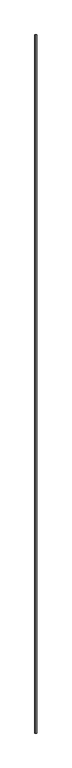
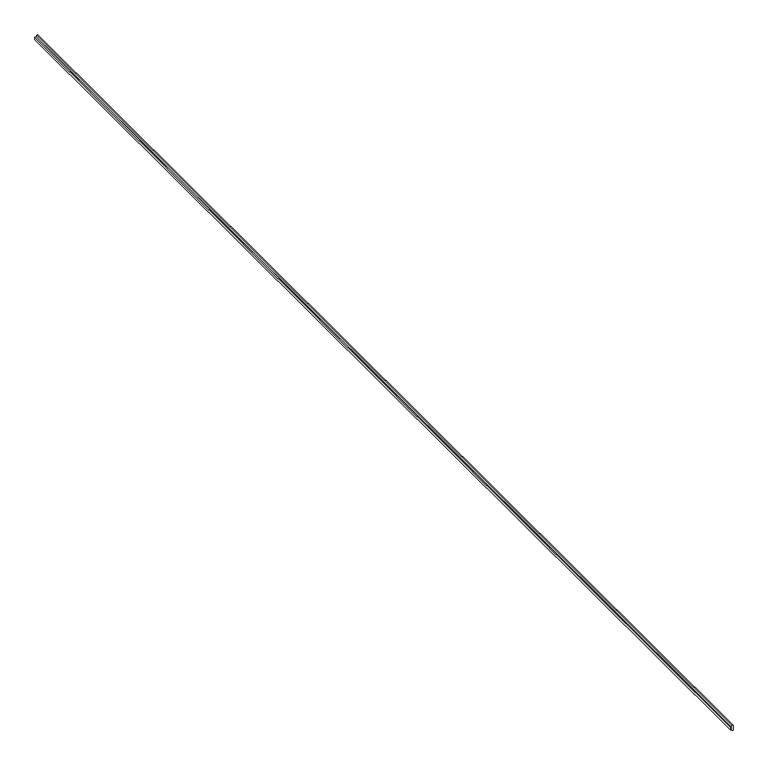
"""IFC4 building model written with IfcOpenShell, lengths in millimetres: proxy geometry, Door frame4:Door frame004:296162 : Door frame4:Door frame004:296162."""

from ifc_helpers import new_model, si_unit, frame, origin, place, context, project, spatial, polyline, outline, extrude, source, transform, mapped, element, save


def generic_models_a1dbba7a(model_context):
    return source(origin(), model_context, "Body", "SweptSolid", [
        extrude(outline(polyline([(36683.9780947, 20302.9683595), (36685.3750947, 20302.9683595), (36685.3750947, 20301.9015595), (36680.8030947, 20301.9015595), (36680.8030947, 20302.9683595), (36682.2000947, 20302.9683595), (36682.2000947, 20304.7463595), (36678.7014343, 20304.7463595), (36678.7014343, 20306.9383326), (36687.4772673, 20306.9383326), (36687.4772673, 20304.7464101), (36683.9780947, 20304.7464101), (36683.9780947, 20302.9683595)])), frame((0.0, -774.5581156, 0.0), z_axis=(0.0, 1.0, 0.0), x_axis=(0.0, 0.0, 1.0)), (0.0, 0.0, 1.0), 1999.85),
    ])


if __name__ == "__main__":
    model = new_model("IFC4")
    model_context = context("Model", 3, world=origin())
    ifc_project = project(units=[si_unit("LENGTHUNIT", "METRE", prefix="MILLI")], contexts=[model_context])
    site = spatial("IfcSite", under=ifc_project)
    building = spatial("IfcBuilding", under=site)
    placement = place(None, origin())
    generic_models_shape = generic_models_a1dbba7a(model_context)
    element("IfcBuildingElementProxy", 1, Name="Door frame4:Door frame004:296162 : Door frame4:Door frame004:296162", ObjectType="Door frame4:Door frame004:296162 : Door frame4:Door frame004:296162", at=placement, inside=building, context=model_context, shape_type="MappedRepresentation", body=[
        mapped(generic_models_shape, transform((0.0, 0.0, 0.0), x_axis=(1.0, 0.0, 0.0), y_axis=(0.0, 1.0, 0.0), z_axis=(0.0, 0.0, 1.0))),
    ])
    save(model, "model.ifc")

# Revit data of these elements
# Type "Door frame4:Door frame004:296162 : Door frame4:Door frame004:296162"
#   NameOverride = "Door frame4:Door frame004:296162"
#   ObjectTypeOverride = "Door frame4:Door frame004"
#   Reference = "Door frame004"
#   Category = "Generic Models"
#   Tag = "296162"
# Element 1 (IfcBuildingElementProxy, "Door frame4:Door frame004:296162 : Door frame4:Door frame004:296162")
#   Materials on its faces: "FLEETWOOD SERIES T-3200 SINGLE SWING DOOR FRAME"
# Materials
#   "FLEETWOOD SERIES T-3200 SINGLE SWING DOOR FRAME": class "Unassigned", colour RGB 128 128 128, transparency 0, Cost = 0
